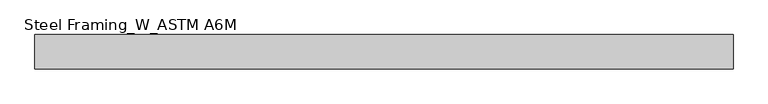
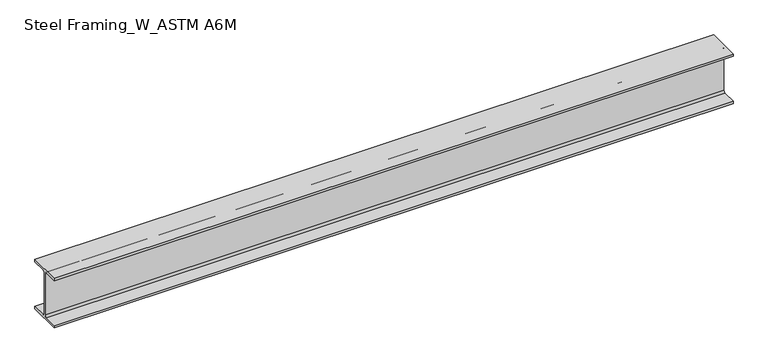
"""IFC4 building model written with IfcOpenShell, lengths in millimetres: beam geometry, Steel Framing_W_ASTM A6M : H_SB_AR_S02_W200x31.3_B6."""

import ifcopenshell
import ifcopenshell.guid

model = None  # the IFC model being written
_history = None  # IfcOwnerHistory: only IFC2X3 demands one
_inside = {}  # id of a spatial element -> (the spatial element, [elements in it])
_under = {}  # id of a project, library or spatial element -> (it, [spatial elements below it])
_declared = {}  # id of a project -> (the project, [libraries it declares])
_typed = {}  # id of a type object -> (the type object, [elements of that type])
_made_of = {}  # id of a material, layer set ... -> (it, [elements and type objects made of it])


def new_model(schema):
    """Start an empty IFC model of exactly this schema.

    Asked for "IFC4X3", IfcOpenShell would pick the latest addendum, in which some entities
    have other attributes; the version numbers below select the first issue.
    IFC2X3 requires an IfcOwnerHistory on every rooted entity: one is made here for all.
    """
    global model, _history
    if schema == "IFC4X3":
        model = ifcopenshell.file(schema_version=(4, 3, 0, 0))
    else:
        model = ifcopenshell.file(schema=schema)
    _inside.clear()
    _under.clear()
    _declared.clear()
    _typed.clear()
    _made_of.clear()
    _history = None
    if model.schema == "IFC2X3":
        org = make("IfcOrganization", Name="unknown")
        user = make(
            "IfcPersonAndOrganization",
            ThePerson=make("IfcPerson", FamilyName="unknown"),
            TheOrganization=org,
        )
        app = make(
            "IfcApplication",
            ApplicationDeveloper=org,
            Version="unknown",
            ApplicationFullName="unknown",
            ApplicationIdentifier="unknown",
        )
        _history = make(
            "IfcOwnerHistory",
            OwningUser=user,
            OwningApplication=app,
            ChangeAction="ADDED",
            CreationDate=0,
        )
    return model


def make(cls, **values):
    """One entity of the class cls with the attributes given. An attribute that is None is left unset."""
    return model.create_entity(
        cls, **{name: value for name, value in values.items() if value is not None}
    )


def rooted(cls, **values):
    """An entity with a GlobalId (a new one), such as an element, a storey or a relation."""
    return make(cls, GlobalId=ifcopenshell.guid.new(), OwnerHistory=_history, **values)


def si_unit(unit_type, name, prefix=None):
    """IfcSIUnit, for example si_unit("LENGTHUNIT", "METRE", prefix="MILLI")."""
    return make("IfcSIUnit", UnitType=unit_type, Prefix=prefix, Name=name)


def assignment(units):
    """IfcUnitAssignment: the units of a project."""
    return None if units is None else make("IfcUnitAssignment", Units=units)


def point(xyz):
    """IfcCartesianPoint."""
    return None if xyz is None else make("IfcCartesianPoint", Coordinates=xyz)


def direction(xyz):
    """IfcDirection."""
    return None if xyz is None else make("IfcDirection", DirectionRatios=xyz)


def frame(location, z_axis=None, x_axis=None):
    """IfcAxis2Placement3D, a coordinate frame: its origin and axes. An axis left out is left unset."""
    return make(
        "IfcAxis2Placement3D",
        Location=point(location),
        Axis=direction(z_axis),
        RefDirection=direction(x_axis),
    )


def frame_2d(location, x_axis=None):
    """IfcAxis2Placement2D, a coordinate frame in the plane: its origin and x axis."""
    return make(
        "IfcAxis2Placement2D", Location=point(location), RefDirection=direction(x_axis)
    )


def origin():
    """The frame at (0, 0, 0) with its axes left unset."""
    return frame((0.0, 0.0, 0.0))


def place(relative_to, where):
    """IfcLocalPlacement: puts the frame where relative to a parent placement (None: the world)."""
    return make(
        "IfcLocalPlacement", PlacementRelTo=relative_to, RelativePlacement=where
    )


def context(
    kind, dimensions, precision=None, world=None, true_north=None, identifier=None
):
    """IfcGeometricRepresentationContext, for example the 3D "Model" context."""
    return make(
        "IfcGeometricRepresentationContext",
        ContextIdentifier=identifier,
        ContextType=kind,
        CoordinateSpaceDimension=dimensions,
        Precision=precision,
        WorldCoordinateSystem=world,
        TrueNorth=true_north,
    )


def project(units=None, contexts=None):
    """IfcProject with its units and contexts."""
    return rooted(
        "IfcProject",
        Name="project",
        RepresentationContexts=contexts,
        UnitsInContext=assignment(units),
    )


def spatial(cls, under=None, at=None, **own):
    """A site, building, storey or space (cls), placed at a placement, below another one or the project."""
    s = rooted(cls, ObjectPlacement=at, **own)
    if under is not None:
        _under.setdefault(under.id(), (under, []))[1].append(s)
    return s


def polyline(points):
    """IfcPolyline through the points."""
    return make("IfcPolyline", Points=[point(p) for p in points])


def circle_curve(where, radius):
    """IfcCircle in the frame where."""
    return make("IfcCircle", Position=where, Radius=radius)


def trimmed(basis, trim1, trim2, sense, master):
    """IfcTrimmedCurve: the piece of a basis curve between two trims."""
    return make(
        "IfcTrimmedCurve",
        BasisCurve=basis,
        Trim1=trim1,
        Trim2=trim2,
        SenseAgreement=sense,
        MasterRepresentation=master,
    )


def segment(curve, same_sense, transition):
    """IfcCompositeCurveSegment."""
    return make(
        "IfcCompositeCurveSegment",
        Transition=transition,
        SameSense=same_sense,
        ParentCurve=curve,
    )


def composite_curve(segments, self_intersect=None):
    """IfcCompositeCurve: segments joined end to end."""
    return make("IfcCompositeCurve", Segments=segments, SelfIntersect=self_intersect)


def outline(outer, holes=None, kind="AREA"):
    """IfcArbitraryClosedProfileDef: a profile drawn as a closed curve; with holes, ...WithVoids."""
    if holes is None:
        return make("IfcArbitraryClosedProfileDef", ProfileType=kind, OuterCurve=outer)
    return make(
        "IfcArbitraryProfileDefWithVoids",
        ProfileType=kind,
        OuterCurve=outer,
        InnerCurves=holes,
    )


def extrude(swept, where, along, depth):
    """IfcExtrudedAreaSolid: the profile swept, set in the frame where, extruded along a direction by depth."""
    return make(
        "IfcExtrudedAreaSolid",
        SweptArea=swept,
        Position=where,
        ExtrudedDirection=direction(along),
        Depth=depth,
    )


def shape(context_of_items, identifier, shape_type, items):
    """IfcShapeRepresentation: the items that make up one representation, for example the "Body"."""
    return make(
        "IfcShapeRepresentation",
        ContextOfItems=context_of_items,
        RepresentationIdentifier=identifier,
        RepresentationType=shape_type,
        Items=items,
    )


def source(mapping_origin, context_of_items, identifier, shape_type, items):
    """IfcRepresentationMap: a shape defined once, which mapped items show again and again."""
    return make(
        "IfcRepresentationMap",
        MappingOrigin=mapping_origin,
        MappedRepresentation=shape(context_of_items, identifier, shape_type, items),
    )


def transform(
    local_origin,
    x_axis=None,
    y_axis=None,
    z_axis=None,
    scale=None,
    scale2=None,
    scale3=None,
    uniform=True,
):
    """IfcCartesianTransformationOperator3D, or its non-uniform kind. x_axis, y_axis, z_axis: its Axis1, 2, 3."""
    if uniform:
        return make(
            "IfcCartesianTransformationOperator3D",
            Axis1=direction(x_axis),
            Axis2=direction(y_axis),
            LocalOrigin=point(local_origin),
            Scale=scale,
            Axis3=direction(z_axis),
        )
    return make(
        "IfcCartesianTransformationOperator3DnonUniform",
        Axis1=direction(x_axis),
        Axis2=direction(y_axis),
        LocalOrigin=point(local_origin),
        Scale=scale,
        Axis3=direction(z_axis),
        Scale2=scale2,
        Scale3=scale3,
    )


def mapped(mapping_source, mapping_target):
    """IfcMappedItem: shows the shape of a source again, moved by a transform."""
    return make(
        "IfcMappedItem", MappingSource=mapping_source, MappingTarget=mapping_target
    )


def made_of(thing, what):
    """Note that an element or type object is made of a material, layer set ...; save() writes the relation."""
    if what is not None:
        _made_of.setdefault(what.id(), (what, []))[1].append(thing)
    return thing


def element(
    cls,
    number,
    at=None,
    inside=None,
    cuts=None,
    type_object=None,
    material=None,
    context=None,
    identifier="Body",
    shape_type=None,
    held_by="IfcProductDefinitionShape",
    body=None,
    shapes=None,
    **own,
):
    """One element of the class cls, such as IfcWall. Its Tag is "e" and its number.

    at: its placement. inside: the storey or other place that contains it. cuts: it is an
    opening in that element (IfcRelVoidsElement). A single representation is given by context,
    identifier, shape_type and body (its items); several are given by shapes. held_by: the class
    of the entity that holds the representations. save() writes the other relations.
    """
    e = rooted(cls, Tag="e%d" % number, ObjectPlacement=at, **own)
    if body is not None:
        shapes = [shape(context, identifier, shape_type, body)]
    if shapes is not None:
        e.Representation = make(held_by, Representations=shapes)
    if inside is not None:
        _inside.setdefault(inside.id(), (inside, []))[1].append(e)
    if cuts is not None:
        rooted(
            "IfcRelVoidsElement", RelatingBuildingElement=cuts, RelatedOpeningElement=e
        )
    if type_object is not None:
        _typed.setdefault(type_object.id(), (type_object, []))[1].append(e)
    return made_of(e, material)


def aggregate(whole, parts):
    """IfcRelAggregates: a whole, such as a stair, and the parts it consists of."""
    return rooted("IfcRelAggregates", RelatingObject=whole, RelatedObjects=parts)


def save(model, path):
    """Write the relations noted so far, then the file.

    IfcRelAggregates (storeys below a building ...), IfcRelContainedInSpatialStructure (elements
    in a storey), IfcRelDefinesByType, IfcRelAssociatesMaterial and IfcRelDeclares: one each for
    every whole, place, type object, material and project.
    """
    for whole, parts in _under.values():
        aggregate(whole, parts)
    for where, things in _inside.values():
        rooted(
            "IfcRelContainedInSpatialStructure",
            RelatedElements=things,
            RelatingStructure=where,
        )
    for kind, things in _typed.values():
        rooted("IfcRelDefinesByType", RelatedObjects=things, RelatingType=kind)
    for what, things in _made_of.values():
        rooted("IfcRelAssociatesMaterial", RelatedObjects=things, RelatingMaterial=what)
    for by, libraries in _declared.values():
        rooted("IfcRelDeclares", RelatingContext=by, RelatedDefinitions=libraries)
    model.write(path)


def steel_framing_w_astm_a6m_9acaacfc(model_context):
    return source(origin(), model_context, "Body", "SweptSolid", [
        extrude(outline(composite_curve([segment(polyline([(67.0, -94.8), (67.0, -105.0), (-67.0, -105.0), (-67.0, -94.8), (-10.775, -94.8)]), True, "CONTINUOUS"), segment(trimmed(circle_curve(frame_2d((-10.775, -87.2)), 7.6), [point((-10.775, -94.8))], [point((-3.175, -87.2))], True, "CARTESIAN"), True, "CONTINUOUS"), segment(polyline([(-3.175, -87.2), (-3.175, 87.2)]), True, "CONTINUOUS"), segment(trimmed(circle_curve(frame_2d((-10.775, 87.2)), 7.6), [point((-3.175, 87.2))], [point((-10.775, 94.8))], True, "CARTESIAN"), True, "CONTINUOUS"), segment(polyline([(-10.775, 94.8), (-67.0, 94.8), (-67.0, 105.0), (67.0, 105.0), (67.0, 94.8), (10.775, 94.8)]), True, "CONTINUOUS"), segment(trimmed(circle_curve(frame_2d((10.775, 87.2)), 7.6), [point((10.775, 94.8))], [point((3.175, 87.2))], True, "CARTESIAN"), True, "CONTINUOUS"), segment(polyline([(3.175, 87.2), (3.175, -87.2)]), True, "CONTINUOUS"), segment(trimmed(circle_curve(frame_2d((10.775, -87.2)), 7.6), [point((3.175, -87.2))], [point((10.775, -94.8))], True, "CARTESIAN"), True, "CONTINUOUS"), segment(polyline([(10.775, -94.8), (67.0, -94.8)]), True, "CONTINUOUS")], self_intersect=False)), frame((-1360.3, 0.0, 0.0), z_axis=(1.0, 0.0, 0.0), x_axis=(0.0, 1.0, 0.0)), (0.0, 0.0, 1.0), 2720.6),
    ])


if __name__ == "__main__":
    model = new_model("IFC4")
    model_context = context("Model", 3, world=origin())
    ifc_project = project(units=[si_unit("LENGTHUNIT", "METRE", prefix="MILLI")], contexts=[model_context])
    site = spatial("IfcSite", under=ifc_project)
    building = spatial("IfcBuilding", under=site)
    placement = place(None, origin())
    steel_framing_w_astm_a6m_shape = steel_framing_w_astm_a6m_9acaacfc(model_context)
    element("IfcBeam", 1, ObjectType="Steel Framing_W_ASTM A6M : H_SB_AR_S02_W200x31.3_B6", at=placement, inside=building, context=model_context, shape_type="MappedRepresentation", body=[
        mapped(steel_framing_w_astm_a6m_shape, transform((0.0, 0.0, 0.0), x_axis=(1.0, 0.0, 0.0), y_axis=(0.0, 1.0, 0.0), z_axis=(0.0, 0.0, 1.0))),
    ])
    save(model, "model.ifc")

# Revit data of these elements
# Type "Steel Framing_W_ASTM A6M : H_SB_AR_S02_W200x31.3_B6"
#   Type Mark = "B6"
#   Section Name Key = "W8x21"
#   Width = 13.4 cm
#   Web Thickness = 0.635 cm
#   Web Fillet = 0.76 cm
#   Warping Constant = 40800.0 cm⁶
#   Torsional Moment of Inertia = 11.70 cm⁴
#   Section Area = 39.7 cm²
#   Plastic Modulus weak axis = 93.2 cm³
#   Plastic Modulus strong axis = 334.0 cm³
#   Perimeter = 0.93 m²/m
#   Nominal Weight = 31.30 kgf/m
#   Moment of Inertia weak axis = 407.00 cm⁴
#   Moment of Inertia strong axis = 3130.00 cm⁴
#   Height = 21.0 cm
#   Flange Thickness = 1.02 cm
#   Elastic Modulus weak axis = 60.8 cm³
#   Elastic Modulus strong axis = 298.0 cm³
#   Centroid Vertical = 10.5 cm
#   Centroid Horizontal = 6.7 cm
#   Length [instance default] = 1500 mm
#   Structural Material [instance default] = Steel, 45-345
#   Bolt Spacing = 0
#   Assembly Code = ""
# Element 1 (IfcBeam, "Steel Framing_W_ASTM A6M : H_SB_AR_S02_W200x31.3_B6")
#   Materials on its faces: "Steel, 45-345"
# Materials
#   "Steel, 45-345": class "Metal", colour RGB 189 187 185, transparency 0, Description = "Steel 345 MPa", Cost = 0
